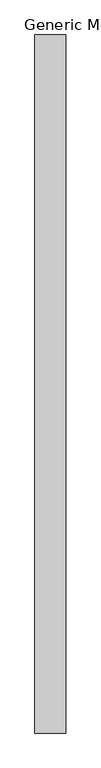
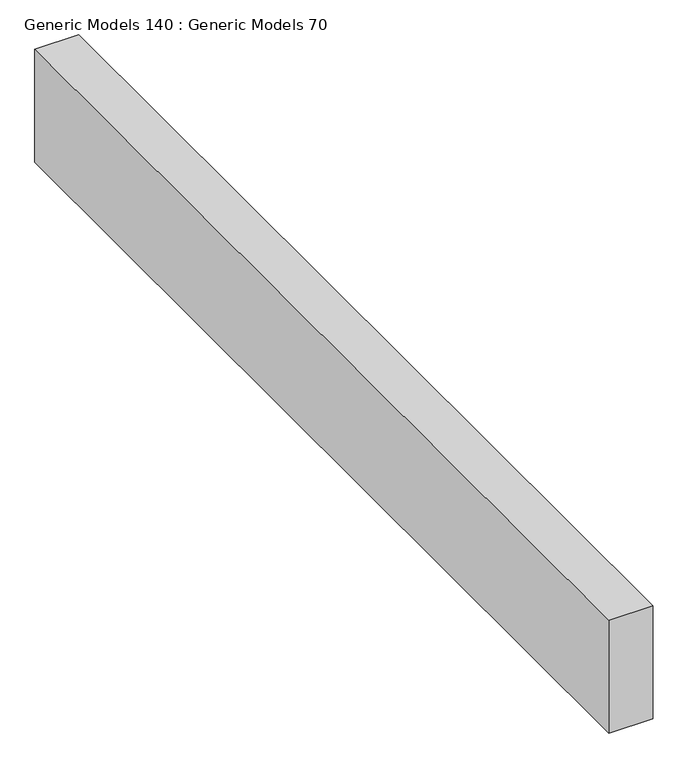
"""IFC4 building model written with IfcOpenShell, lengths in millimetres: proxy geometry, Generic Models 140 : Generic Models 70."""

import ifcopenshell
import ifcopenshell.guid

model = None  # the IFC model being written
_history = None  # IfcOwnerHistory: only IFC2X3 demands one
_inside = {}  # id of a spatial element -> (the spatial element, [elements in it])
_under = {}  # id of a project, library or spatial element -> (it, [spatial elements below it])
_declared = {}  # id of a project -> (the project, [libraries it declares])
_typed = {}  # id of a type object -> (the type object, [elements of that type])
_made_of = {}  # id of a material, layer set ... -> (it, [elements and type objects made of it])


def new_model(schema):
    """Start an empty IFC model of exactly this schema.

    Asked for "IFC4X3", IfcOpenShell would pick the latest addendum, in which some entities
    have other attributes; the version numbers below select the first issue.
    IFC2X3 requires an IfcOwnerHistory on every rooted entity: one is made here for all.
    """
    global model, _history
    if schema == "IFC4X3":
        model = ifcopenshell.file(schema_version=(4, 3, 0, 0))
    else:
        model = ifcopenshell.file(schema=schema)
    _inside.clear()
    _under.clear()
    _declared.clear()
    _typed.clear()
    _made_of.clear()
    _history = None
    if model.schema == "IFC2X3":
        org = make("IfcOrganization", Name="unknown")
        user = make(
            "IfcPersonAndOrganization",
            ThePerson=make("IfcPerson", FamilyName="unknown"),
            TheOrganization=org,
        )
        app = make(
            "IfcApplication",
            ApplicationDeveloper=org,
            Version="unknown",
            ApplicationFullName="unknown",
            ApplicationIdentifier="unknown",
        )
        _history = make(
            "IfcOwnerHistory",
            OwningUser=user,
            OwningApplication=app,
            ChangeAction="ADDED",
            CreationDate=0,
        )
    return model


def make(cls, **values):
    """One entity of the class cls with the attributes given. An attribute that is None is left unset."""
    return model.create_entity(
        cls, **{name: value for name, value in values.items() if value is not None}
    )


def rooted(cls, **values):
    """An entity with a GlobalId (a new one), such as an element, a storey or a relation."""
    return make(cls, GlobalId=ifcopenshell.guid.new(), OwnerHistory=_history, **values)


def si_unit(unit_type, name, prefix=None):
    """IfcSIUnit, for example si_unit("LENGTHUNIT", "METRE", prefix="MILLI")."""
    return make("IfcSIUnit", UnitType=unit_type, Prefix=prefix, Name=name)


def assignment(units):
    """IfcUnitAssignment: the units of a project."""
    return None if units is None else make("IfcUnitAssignment", Units=units)


def point(xyz):
    """IfcCartesianPoint."""
    return None if xyz is None else make("IfcCartesianPoint", Coordinates=xyz)


def direction(xyz):
    """IfcDirection."""
    return None if xyz is None else make("IfcDirection", DirectionRatios=xyz)


def frame(location, z_axis=None, x_axis=None):
    """IfcAxis2Placement3D, a coordinate frame: its origin and axes. An axis left out is left unset."""
    return make(
        "IfcAxis2Placement3D",
        Location=point(location),
        Axis=direction(z_axis),
        RefDirection=direction(x_axis),
    )


def origin():
    """The frame at (0, 0, 0) with its axes left unset."""
    return frame((0.0, 0.0, 0.0))


def place(relative_to, where):
    """IfcLocalPlacement: puts the frame where relative to a parent placement (None: the world)."""
    return make(
        "IfcLocalPlacement", PlacementRelTo=relative_to, RelativePlacement=where
    )


def context(
    kind, dimensions, precision=None, world=None, true_north=None, identifier=None
):
    """IfcGeometricRepresentationContext, for example the 3D "Model" context."""
    return make(
        "IfcGeometricRepresentationContext",
        ContextIdentifier=identifier,
        ContextType=kind,
        CoordinateSpaceDimension=dimensions,
        Precision=precision,
        WorldCoordinateSystem=world,
        TrueNorth=true_north,
    )


def project(units=None, contexts=None):
    """IfcProject with its units and contexts."""
    return rooted(
        "IfcProject",
        Name="project",
        RepresentationContexts=contexts,
        UnitsInContext=assignment(units),
    )


def spatial(cls, under=None, at=None, **own):
    """A site, building, storey or space (cls), placed at a placement, below another one or the project."""
    s = rooted(cls, ObjectPlacement=at, **own)
    if under is not None:
        _under.setdefault(under.id(), (under, []))[1].append(s)
    return s


def polyline(points):
    """IfcPolyline through the points."""
    return make("IfcPolyline", Points=[point(p) for p in points])


def outline(outer, holes=None, kind="AREA"):
    """IfcArbitraryClosedProfileDef: a profile drawn as a closed curve; with holes, ...WithVoids."""
    if holes is None:
        return make("IfcArbitraryClosedProfileDef", ProfileType=kind, OuterCurve=outer)
    return make(
        "IfcArbitraryProfileDefWithVoids",
        ProfileType=kind,
        OuterCurve=outer,
        InnerCurves=holes,
    )


def extrude(swept, where, along, depth):
    """IfcExtrudedAreaSolid: the profile swept, set in the frame where, extruded along a direction by depth."""
    return make(
        "IfcExtrudedAreaSolid",
        SweptArea=swept,
        Position=where,
        ExtrudedDirection=direction(along),
        Depth=depth,
    )


def shape(context_of_items, identifier, shape_type, items):
    """IfcShapeRepresentation: the items that make up one representation, for example the "Body"."""
    return make(
        "IfcShapeRepresentation",
        ContextOfItems=context_of_items,
        RepresentationIdentifier=identifier,
        RepresentationType=shape_type,
        Items=items,
    )


def source(mapping_origin, context_of_items, identifier, shape_type, items):
    """IfcRepresentationMap: a shape defined once, which mapped items show again and again."""
    return make(
        "IfcRepresentationMap",
        MappingOrigin=mapping_origin,
        MappedRepresentation=shape(context_of_items, identifier, shape_type, items),
    )


def transform(
    local_origin,
    x_axis=None,
    y_axis=None,
    z_axis=None,
    scale=None,
    scale2=None,
    scale3=None,
    uniform=True,
):
    """IfcCartesianTransformationOperator3D, or its non-uniform kind. x_axis, y_axis, z_axis: its Axis1, 2, 3."""
    if uniform:
        return make(
            "IfcCartesianTransformationOperator3D",
            Axis1=direction(x_axis),
            Axis2=direction(y_axis),
            LocalOrigin=point(local_origin),
            Scale=scale,
            Axis3=direction(z_axis),
        )
    return make(
        "IfcCartesianTransformationOperator3DnonUniform",
        Axis1=direction(x_axis),
        Axis2=direction(y_axis),
        LocalOrigin=point(local_origin),
        Scale=scale,
        Axis3=direction(z_axis),
        Scale2=scale2,
        Scale3=scale3,
    )


def mapped(mapping_source, mapping_target):
    """IfcMappedItem: shows the shape of a source again, moved by a transform."""
    return make(
        "IfcMappedItem", MappingSource=mapping_source, MappingTarget=mapping_target
    )


def made_of(thing, what):
    """Note that an element or type object is made of a material, layer set ...; save() writes the relation."""
    if what is not None:
        _made_of.setdefault(what.id(), (what, []))[1].append(thing)
    return thing


def element(
    cls,
    number,
    at=None,
    inside=None,
    cuts=None,
    type_object=None,
    material=None,
    context=None,
    identifier="Body",
    shape_type=None,
    held_by="IfcProductDefinitionShape",
    body=None,
    shapes=None,
    **own,
):
    """One element of the class cls, such as IfcWall. Its Tag is "e" and its number.

    at: its placement. inside: the storey or other place that contains it. cuts: it is an
    opening in that element (IfcRelVoidsElement). A single representation is given by context,
    identifier, shape_type and body (its items); several are given by shapes. held_by: the class
    of the entity that holds the representations. save() writes the other relations.
    """
    e = rooted(cls, Tag="e%d" % number, ObjectPlacement=at, **own)
    if body is not None:
        shapes = [shape(context, identifier, shape_type, body)]
    if shapes is not None:
        e.Representation = make(held_by, Representations=shapes)
    if inside is not None:
        _inside.setdefault(inside.id(), (inside, []))[1].append(e)
    if cuts is not None:
        rooted(
            "IfcRelVoidsElement", RelatingBuildingElement=cuts, RelatedOpeningElement=e
        )
    if type_object is not None:
        _typed.setdefault(type_object.id(), (type_object, []))[1].append(e)
    return made_of(e, material)


def aggregate(whole, parts):
    """IfcRelAggregates: a whole, such as a stair, and the parts it consists of."""
    return rooted("IfcRelAggregates", RelatingObject=whole, RelatedObjects=parts)


def save(model, path):
    """Write the relations noted so far, then the file.

    IfcRelAggregates (storeys below a building ...), IfcRelContainedInSpatialStructure (elements
    in a storey), IfcRelDefinesByType, IfcRelAssociatesMaterial and IfcRelDeclares: one each for
    every whole, place, type object, material and project.
    """
    for whole, parts in _under.values():
        aggregate(whole, parts)
    for where, things in _inside.values():
        rooted(
            "IfcRelContainedInSpatialStructure",
            RelatedElements=things,
            RelatingStructure=where,
        )
    for kind, things in _typed.values():
        rooted("IfcRelDefinesByType", RelatedObjects=things, RelatingType=kind)
    for what, things in _made_of.values():
        rooted("IfcRelAssociatesMaterial", RelatedObjects=things, RelatingMaterial=what)
    for by, libraries in _declared.values():
        rooted("IfcRelDeclares", RelatingContext=by, RelatedDefinitions=libraries)
    model.write(path)


def generic_models_140_generic_models_70_87271439(model_context):
    return source(origin(), model_context, "Body", "SweptSolid", [
        extrude(outline(polyline([(32200.8585525, 39663.9958903), (32200.8585525, 36493.1457942), (32061.1585525, 36493.1457942), (32061.1585525, 39663.9958903), (32200.8585525, 39663.9958903)])), frame((0.0, 0.0, 268757.4), z_axis=(0.0, 0.0, 1.0), x_axis=(1.0, 0.0, 0.0)), (0.0, 0.0, 1.0), 381.0),
    ])


if __name__ == "__main__":
    model = new_model("IFC4")
    model_context = context("Model", 3, world=origin())
    ifc_project = project(units=[si_unit("LENGTHUNIT", "METRE", prefix="MILLI")], contexts=[model_context])
    site = spatial("IfcSite", under=ifc_project)
    building = spatial("IfcBuilding", under=site)
    placement = place(None, origin())
    generic_models_140_generic_models_70_shape = generic_models_140_generic_models_70_87271439(model_context)
    element("IfcBuildingElementProxy", 1, Name="Generic Models 140 : Generic Models 70", ObjectType="Generic Models 140 : Generic Models 70", at=placement, inside=building, context=model_context, shape_type="MappedRepresentation", body=[
        mapped(generic_models_140_generic_models_70_shape, transform((0.0, 0.0, 0.0), x_axis=(1.0, 0.0, 0.0), y_axis=(0.0, 1.0, 0.0), z_axis=(0.0, 0.0, 1.0))),
    ])
    save(model, "model.ifc")

# Revit data of these elements
# Element 1 (IfcBuildingElementProxy, "Generic Models 140 : Generic Models 70")
#   Materials on its faces: "3 1/2\" x 15\" GLUELAM BEAM"
# Materials
#   "3 1/2\" x 15\" GLUELAM BEAM": class "Wood", colour RGB 214 169 150, transparency 0, Description = "Pinus Echinata", Cost = 0
